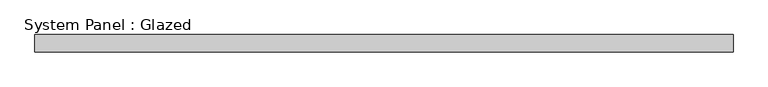
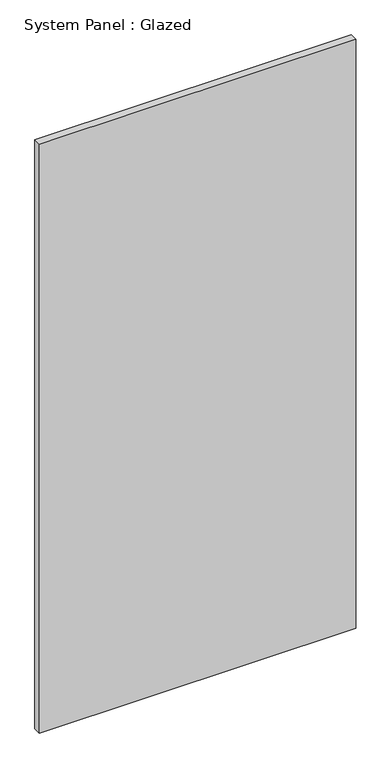
"""IFC4 building model written with IfcOpenShell, lengths in millimetres: plate geometry, System Panel : Glazed."""

from ifc_helpers import new_model, si_unit, origin, origin_with_axes, place, context, project, spatial, polyline, outline, extrude, source, transform, mapped, element, save


def system_panel_glazed_816bae74(model_context):
    return source(origin(), model_context, "Body", "SweptSolid", [
        extrude(outline(polyline([(507.8156411, 24.5), (-507.8156411, 24.5), (-507.8156411, 49.5), (507.8156411, 49.5), (507.8156411, 24.5)])), origin_with_axes(), (0.0, 0.0, 1.0), 2000.0),
    ])


if __name__ == "__main__":
    model = new_model("IFC4")
    model_context = context("Model", 3, world=origin())
    ifc_project = project(units=[si_unit("LENGTHUNIT", "METRE", prefix="MILLI")], contexts=[model_context])
    site = spatial("IfcSite", under=ifc_project)
    building = spatial("IfcBuilding", under=site)
    placement = place(None, origin())
    system_panel_glazed_shape = system_panel_glazed_816bae74(model_context)
    element("IfcPlate", 1, ObjectType="System Panel : Glazed", at=placement, inside=building, context=model_context, shape_type="MappedRepresentation", body=[
        mapped(system_panel_glazed_shape, transform((0.0, 0.0, 0.0), x_axis=(1.0, 0.0, 0.0), y_axis=(0.0, 1.0, 0.0), z_axis=(0.0, 0.0, 1.0))),
    ])
    save(model, "model.ifc")

# Revit data of these elements
# Element 1 (IfcPlate, "System Panel : Glazed")
#   Materials on its faces: "Glass"
# Materials
#   "Glass": class "Glass", colour RGB 218 227 224, transparency 0.85, Description = "Soda Lime Glass", Cost = 0
